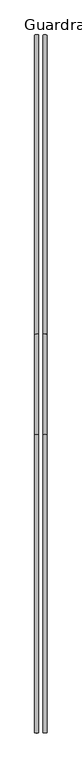
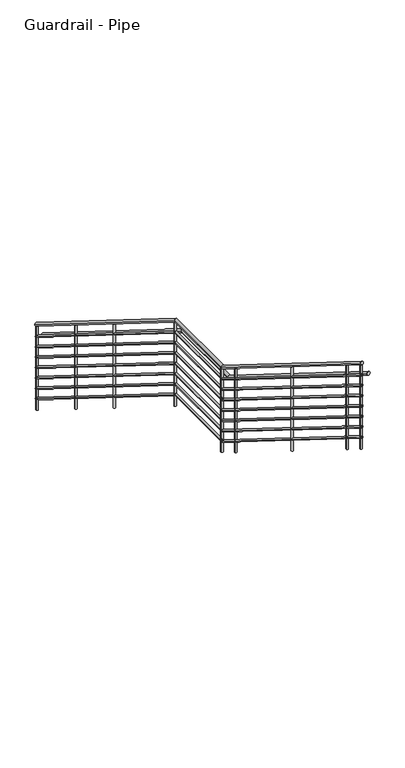
"""IFC4 building model written with IfcOpenShell, lengths in millimetres: railing geometry, Guardrail - Pipe."""

from ifc_helpers import new_model, si_unit, point, frame, frame_2d, origin, place, context, project, spatial, circle_curve, ellipse_curve, trimmed, segment, composite_curve, outline, extrude, source, transform, mapped, element, save
from ifc_brep_helpers import plane_surface, cylinder_surface, advanced_brep


def guardrail_pipe_06b17180(model_context):
    return source(origin(), model_context, "Body", "SolidModel", [
        advanced_brep(
        [(-3343.0939612, 2884.909643, -2439.0768639), (-3304.9939612, 2884.909643, -2439.0768639), (-3343.0939612, 85.4582154, -693.9642857), (-3304.9939612, 85.4582154, -693.9642857), (-3343.0939612, -854.3417846, -693.9642857), (-3304.9939612, -854.3417846, -693.9642857), (-3343.0939612, -3642.890357, 1044.3517075), (-3304.9939612, -3642.890357, 1044.3517075)],
        [
            (0, 1, ellipse_curve(frame((-3324.0439612, 2884.909643, -2439.0768639), z_axis=(0.0, 1.0, 0.0), x_axis=(0.0, 0.0, -1.0)), 22.4482925, 19.05)),
            (1, 0, ellipse_curve(frame((-3324.0439612, 2884.909643, -2439.0768639), z_axis=(0.0, 1.0, 0.0), x_axis=(0.0, 0.0, -1.0)), 22.4482925, 19.05)),
            (0, 2),
            (2, 3, ellipse_curve(frame((-3324.0439612, 85.4582154, -693.9642857), z_axis=(0.0, 0.9614096116045893, -0.2751209892289441), x_axis=(0.0, -0.27512098922894396, -0.9614096116045893)), 19.8146552, 19.05)),
            (3, 1),
            (3, 2, ellipse_curve(frame((-3324.0439612, 85.4582154, -693.9642857), z_axis=(0.0, 0.9614096116045893, -0.2751209892289441), x_axis=(0.0, -0.27512098922894396, -0.9614096116045893)), 19.8146552, 19.05)),
            (2, 4),
            (4, 5, ellipse_curve(frame((-3324.0439612, -854.3417846, -693.9642857), z_axis=(0.0, 0.9614096116045892, -0.27512098922894423), x_axis=(0.0, 0.2751209892289447, 0.9614096116045893)), 19.8146552, 19.05)),
            (5, 3),
            (5, 4, ellipse_curve(frame((-3324.0439612, -854.3417846, -693.9642857), z_axis=(0.0, 0.9614096116045892, -0.27512098922894423), x_axis=(0.0, 0.2751209892289447, 0.9614096116045893)), 19.8146552, 19.05)),
            (6, 7, ellipse_curve(frame((-3324.0439612, -3642.890357, 1044.3517075), z_axis=(0.0, -1.0, 0.0), x_axis=(0.0, 0.0, -1.0)), 22.4482925, 19.05)),
            (7, 6, ellipse_curve(frame((-3324.0439612, -3642.890357, 1044.3517075), z_axis=(0.0, -1.0, 0.0), x_axis=(0.0, 0.0, -1.0)), 22.4482925, 19.05)),
            (4, 6),
            (7, 5),
        ],
        [
            plane_surface(frame((-3324.0439612, 2884.909643, -2416.6285714), z_axis=(0.0, 1.0, 0.0), x_axis=(0.0, 0.0, -1.0))),
            cylinder_surface(frame((-3324.0439612, 2874.832042, -2432.794723), z_axis=(0.0, 0.8486168825713745, -0.5290079267977392), x_axis=(1.0, 0.0, 0.0)), 19.05),
            cylinder_surface(frame((-3324.0439612, 90.909643, -693.9642857), z_axis=(0.0, 1.0, 0.0), x_axis=(1.0, 0.0, 0.0)), 19.05),
            plane_surface(frame((-3324.0439612, -3642.890357, 1066.8), z_axis=(0.0, -1.0, 0.0), x_axis=(0.0, 0.0, -1.0))),
            cylinder_surface(frame((-3324.0439612, -858.967958, -691.0804373), z_axis=(0.0, 0.8486168825713742, -0.5290079267977394), x_axis=(1.0, 0.0, 0.0)), 19.05),
        ],
        [
            (0, [[1, 2]]),
            (1, [[-1, 3, 4, 5]]),
            (1, [[-2, -5, 6, -3]]),
            (2, [[-4, 7, 8, 9]]),
            (2, [[-6, -9, 10, -7]]),
            (3, [[11, 12]]),
            (4, [[-8, 13, -12, 14]]),
            (4, [[-10, -14, -11, -13]]),
        ],
    ),
        advanced_brep(
        [(-3336.7439612, 2884.909643, -2583.9940998), (-3311.3439612, 2884.909643, -2583.9940998), (-3336.7439612, 87.2753579, -840.0142857), (-3311.3439612, 87.2753579, -840.0142857), (-3336.7439612, -852.5246421, -840.0142857), (-3311.3439612, -852.5246421, -840.0142857), (-3336.7439612, -3642.890357, 899.4344717), (-3311.3439612, -3642.890357, 899.4344717)],
        [
            (0, 1, ellipse_curve(frame((-3324.0439612, 2884.909643, -2583.9940998), z_axis=(0.0, 1.0, 0.0), x_axis=(0.0, 0.0, -1.0)), 14.9655283, 12.7)),
            (1, 0, ellipse_curve(frame((-3324.0439612, 2884.909643, -2583.9940998), z_axis=(0.0, 1.0, 0.0), x_axis=(0.0, 0.0, -1.0)), 14.9655283, 12.7)),
            (0, 2),
            (2, 3, ellipse_curve(frame((-3324.0439612, 87.2753579, -840.0142857), z_axis=(0.0, 0.9614096116045893, -0.2751209892289441), x_axis=(0.0, -0.27512098922894396, -0.9614096116045893)), 13.2097702, 12.7)),
            (3, 1),
            (3, 2, ellipse_curve(frame((-3324.0439612, 87.2753579, -840.0142857), z_axis=(0.0, 0.9614096116045893, -0.2751209892289441), x_axis=(0.0, -0.27512098922894396, -0.9614096116045893)), 13.2097702, 12.7)),
            (2, 4),
            (4, 5, ellipse_curve(frame((-3324.0439612, -852.5246421, -840.0142857), z_axis=(0.0, 0.9614096116045892, -0.27512098922894423), x_axis=(0.0, 0.2751209892289447, 0.9614096116045893)), 13.2097702, 12.7)),
            (5, 3),
            (5, 4, ellipse_curve(frame((-3324.0439612, -852.5246421, -840.0142857), z_axis=(0.0, 0.9614096116045892, -0.27512098922894423), x_axis=(0.0, 0.2751209892289447, 0.9614096116045893)), 13.2097702, 12.7)),
            (6, 7, ellipse_curve(frame((-3324.0439612, -3642.890357, 899.4344717), z_axis=(0.0, -1.0, 0.0), x_axis=(0.0, 0.0, -1.0)), 14.9655283, 12.7)),
            (7, 6, ellipse_curve(frame((-3324.0439612, -3642.890357, 899.4344717), z_axis=(0.0, -1.0, 0.0), x_axis=(0.0, 0.0, -1.0)), 14.9655283, 12.7)),
            (4, 6),
            (7, 5),
        ],
        [
            plane_surface(frame((-3324.0439612, 2884.909643, -2569.0285714), z_axis=(0.0, 1.0, 0.0), x_axis=(0.0, 0.0, -1.0))),
            cylinder_surface(frame((-3324.0439612, 2878.1912423, -2579.8060058), z_axis=(0.0, 0.8486168825713745, -0.5290079267977392), x_axis=(1.0, 0.0, 0.0)), 12.7),
            cylinder_surface(frame((-3324.0439612, 90.909643, -840.0142857), z_axis=(0.0, 1.0, 0.0), x_axis=(1.0, 0.0, 0.0)), 12.7),
            plane_surface(frame((-3324.0439612, -3642.890357, 914.4), z_axis=(0.0, -1.0, 0.0), x_axis=(0.0, 0.0, -1.0))),
            cylinder_surface(frame((-3324.0439612, -855.6087577, -838.0917201), z_axis=(0.0, 0.8486168825713742, -0.5290079267977394), x_axis=(1.0, 0.0, 0.0)), 12.7),
        ],
        [
            (0, [[1, 2]]),
            (1, [[-1, 3, 4, 5]]),
            (1, [[-2, -5, 6, -3]]),
            (2, [[-4, 7, 8, 9]]),
            (2, [[-6, -9, 10, -7]]),
            (3, [[11, 12]]),
            (4, [[-8, 13, -12, 14]]),
            (4, [[-10, -14, -11, -13]]),
        ],
    ),
        advanced_brep(
        [(-3266.8939612, 2884.909643, -2591.4768639), (-3228.7939612, 2884.909643, -2591.4768639), (-3266.8939612, 85.4582154, -846.3642857), (-3228.7939612, 85.4582154, -846.3642857), (-3266.8939612, -854.3417846, -846.3642857), (-3228.7939612, -854.3417846, -846.3642857), (-3266.8939612, -3642.890357, 891.9517075), (-3228.7939612, -3642.890357, 891.9517075)],
        [
            (0, 1, ellipse_curve(frame((-3247.8439612, 2884.909643, -2591.4768639), z_axis=(0.0, 1.0, 0.0), x_axis=(0.0, 0.0, -1.0)), 22.4482925, 19.05)),
            (1, 0, ellipse_curve(frame((-3247.8439612, 2884.909643, -2591.4768639), z_axis=(0.0, 1.0, 0.0), x_axis=(0.0, 0.0, -1.0)), 22.4482925, 19.05)),
            (0, 2),
            (2, 3, ellipse_curve(frame((-3247.8439612, 85.4582154, -846.3642857), z_axis=(0.0, 0.9614096116045893, -0.2751209892289441), x_axis=(0.0, -0.27512098922894396, -0.9614096116045893)), 19.8146552, 19.05)),
            (3, 1),
            (3, 2, ellipse_curve(frame((-3247.8439612, 85.4582154, -846.3642857), z_axis=(0.0, 0.9614096116045893, -0.2751209892289441), x_axis=(0.0, -0.27512098922894396, -0.9614096116045893)), 19.8146552, 19.05)),
            (2, 4),
            (4, 5, ellipse_curve(frame((-3247.8439612, -854.3417846, -846.3642857), z_axis=(0.0, 0.9614096116045892, -0.27512098922894423), x_axis=(0.0, 0.2751209892289447, 0.9614096116045893)), 19.8146552, 19.05)),
            (5, 3),
            (5, 4, ellipse_curve(frame((-3247.8439612, -854.3417846, -846.3642857), z_axis=(0.0, 0.9614096116045892, -0.27512098922894423), x_axis=(0.0, 0.2751209892289447, 0.9614096116045893)), 19.8146552, 19.05)),
            (6, 7, ellipse_curve(frame((-3247.8439612, -3642.890357, 891.9517075), z_axis=(0.0, -1.0, 0.0), x_axis=(0.0, 0.0, -1.0)), 22.4482925, 19.05)),
            (7, 6, ellipse_curve(frame((-3247.8439612, -3642.890357, 891.9517075), z_axis=(0.0, -1.0, 0.0), x_axis=(0.0, 0.0, -1.0)), 22.4482925, 19.05)),
            (4, 6),
            (7, 5),
        ],
        [
            plane_surface(frame((-3247.8439612, 2884.909643, -2569.0285714), z_axis=(0.0, 1.0, 0.0), x_axis=(0.0, 0.0, -1.0))),
            cylinder_surface(frame((-3247.8439612, 2874.832042, -2585.194723), z_axis=(0.0, 0.8486168825713745, -0.5290079267977392), x_axis=(1.0, 0.0, 0.0)), 19.05),
            cylinder_surface(frame((-3247.8439612, 90.909643, -846.3642857), z_axis=(0.0, 1.0, 0.0), x_axis=(1.0, 0.0, 0.0)), 19.05),
            plane_surface(frame((-3247.8439612, -3642.890357, 914.4), z_axis=(0.0, -1.0, 0.0), x_axis=(0.0, 0.0, -1.0))),
            cylinder_surface(frame((-3247.8439612, -858.967958, -843.4804373), z_axis=(0.0, 0.8486168825713742, -0.5290079267977394), x_axis=(1.0, 0.0, 0.0)), 19.05),
        ],
        [
            (0, [[1, 2]]),
            (1, [[-1, 3, 4, 5]]),
            (1, [[-2, -5, 6, -3]]),
            (2, [[-4, 7, 8, 9]]),
            (2, [[-6, -9, 10, -7]]),
            (3, [[11, 12]]),
            (4, [[-8, 13, -12, 14]]),
            (4, [[-10, -14, -11, -13]]),
        ],
    ),
        advanced_brep(
        [(-3336.7439612, 2884.909643, -2710.9940998), (-3311.3439612, 2884.909643, -2710.9940998), (-3336.7439612, 87.2753579, -967.0142857), (-3311.3439612, 87.2753579, -967.0142857), (-3336.7439612, -852.5246421, -967.0142857), (-3311.3439612, -852.5246421, -967.0142857), (-3336.7439612, -3642.890357, 772.4344717), (-3311.3439612, -3642.890357, 772.4344717)],
        [
            (0, 1, ellipse_curve(frame((-3324.0439612, 2884.909643, -2710.9940998), z_axis=(0.0, 1.0, 0.0), x_axis=(0.0, 0.0, -1.0)), 14.9655283, 12.7)),
            (1, 0, ellipse_curve(frame((-3324.0439612, 2884.909643, -2710.9940998), z_axis=(0.0, 1.0, 0.0), x_axis=(0.0, 0.0, -1.0)), 14.9655283, 12.7)),
            (0, 2),
            (2, 3, ellipse_curve(frame((-3324.0439612, 87.2753579, -967.0142857), z_axis=(0.0, 0.9614096116045893, -0.2751209892289441), x_axis=(0.0, -0.27512098922894396, -0.9614096116045893)), 13.2097702, 12.7)),
            (3, 1),
            (3, 2, ellipse_curve(frame((-3324.0439612, 87.2753579, -967.0142857), z_axis=(0.0, 0.9614096116045893, -0.2751209892289441), x_axis=(0.0, -0.27512098922894396, -0.9614096116045893)), 13.2097702, 12.7)),
            (2, 4),
            (4, 5, ellipse_curve(frame((-3324.0439612, -852.5246421, -967.0142857), z_axis=(0.0, 0.9614096116045892, -0.27512098922894423), x_axis=(0.0, 0.2751209892289447, 0.9614096116045893)), 13.2097702, 12.7)),
            (5, 3),
            (5, 4, ellipse_curve(frame((-3324.0439612, -852.5246421, -967.0142857), z_axis=(0.0, 0.9614096116045892, -0.27512098922894423), x_axis=(0.0, 0.2751209892289447, 0.9614096116045893)), 13.2097702, 12.7)),
            (6, 7, ellipse_curve(frame((-3324.0439612, -3642.890357, 772.4344717), z_axis=(0.0, -1.0, 0.0), x_axis=(0.0, 0.0, -1.0)), 14.9655283, 12.7)),
            (7, 6, ellipse_curve(frame((-3324.0439612, -3642.890357, 772.4344717), z_axis=(0.0, -1.0, 0.0), x_axis=(0.0, 0.0, -1.0)), 14.9655283, 12.7)),
            (4, 6),
            (7, 5),
        ],
        [
            plane_surface(frame((-3324.0439612, 2884.909643, -2696.0285714), z_axis=(0.0, 1.0, 0.0), x_axis=(0.0, 0.0, -1.0))),
            cylinder_surface(frame((-3324.0439612, 2878.1912423, -2706.8060058), z_axis=(0.0, 0.8486168825713745, -0.5290079267977392), x_axis=(1.0, 0.0, 0.0)), 12.7),
            cylinder_surface(frame((-3324.0439612, 90.909643, -967.0142857), z_axis=(0.0, 1.0, 0.0), x_axis=(1.0, 0.0, 0.0)), 12.7),
            plane_surface(frame((-3324.0439612, -3642.890357, 787.4), z_axis=(0.0, -1.0, 0.0), x_axis=(0.0, 0.0, -1.0))),
            cylinder_surface(frame((-3324.0439612, -855.6087577, -965.0917201), z_axis=(0.0, 0.8486168825713742, -0.5290079267977394), x_axis=(1.0, 0.0, 0.0)), 12.7),
        ],
        [
            (0, [[1, 2]]),
            (1, [[-1, 3, 4, 5]]),
            (1, [[-2, -5, 6, -3]]),
            (2, [[-4, 7, 8, 9]]),
            (2, [[-6, -9, 10, -7]]),
            (3, [[11, 12]]),
            (4, [[-8, 13, -12, 14]]),
            (4, [[-10, -14, -11, -13]]),
        ],
    ),
        advanced_brep(
        [(-3336.7439612, 2884.909643, -2837.9940998), (-3311.3439612, 2884.909643, -2837.9940998), (-3336.7439612, 87.2753579, -1094.0142857), (-3311.3439612, 87.2753579, -1094.0142857), (-3336.7439612, -852.5246421, -1094.0142857), (-3311.3439612, -852.5246421, -1094.0142857), (-3336.7439612, -3642.890357, 645.4344717), (-3311.3439612, -3642.890357, 645.4344717)],
        [
            (0, 1, ellipse_curve(frame((-3324.0439612, 2884.909643, -2837.9940998), z_axis=(0.0, 1.0, 0.0), x_axis=(0.0, 0.0, -1.0)), 14.9655283, 12.7)),
            (1, 0, ellipse_curve(frame((-3324.0439612, 2884.909643, -2837.9940998), z_axis=(0.0, 1.0, 0.0), x_axis=(0.0, 0.0, -1.0)), 14.9655283, 12.7)),
            (0, 2),
            (2, 3, ellipse_curve(frame((-3324.0439612, 87.2753579, -1094.0142857), z_axis=(0.0, 0.9614096116045893, -0.2751209892289441), x_axis=(0.0, -0.27512098922894396, -0.9614096116045893)), 13.2097702, 12.7)),
            (3, 1),
            (3, 2, ellipse_curve(frame((-3324.0439612, 87.2753579, -1094.0142857), z_axis=(0.0, 0.9614096116045893, -0.2751209892289441), x_axis=(0.0, -0.27512098922894396, -0.9614096116045893)), 13.2097702, 12.7)),
            (2, 4),
            (4, 5, ellipse_curve(frame((-3324.0439612, -852.5246421, -1094.0142857), z_axis=(0.0, 0.9614096116045892, -0.27512098922894423), x_axis=(0.0, 0.2751209892289447, 0.9614096116045893)), 13.2097702, 12.7)),
            (5, 3),
            (5, 4, ellipse_curve(frame((-3324.0439612, -852.5246421, -1094.0142857), z_axis=(0.0, 0.9614096116045892, -0.27512098922894423), x_axis=(0.0, 0.2751209892289447, 0.9614096116045893)), 13.2097702, 12.7)),
            (6, 7, ellipse_curve(frame((-3324.0439612, -3642.890357, 645.4344717), z_axis=(0.0, -1.0, 0.0), x_axis=(0.0, 0.0, -1.0)), 14.9655283, 12.7)),
            (7, 6, ellipse_curve(frame((-3324.0439612, -3642.890357, 645.4344717), z_axis=(0.0, -1.0, 0.0), x_axis=(0.0, 0.0, -1.0)), 14.9655283, 12.7)),
            (4, 6),
            (7, 5),
        ],
        [
            plane_surface(frame((-3324.0439612, 2884.909643, -2823.0285714), z_axis=(0.0, 1.0, 0.0), x_axis=(0.0, 0.0, -1.0))),
            cylinder_surface(frame((-3324.0439612, 2878.1912423, -2833.8060058), z_axis=(0.0, 0.8486168825713745, -0.5290079267977392), x_axis=(1.0, 0.0, 0.0)), 12.7),
            cylinder_surface(frame((-3324.0439612, 90.909643, -1094.0142857), z_axis=(0.0, 1.0, 0.0), x_axis=(1.0, 0.0, 0.0)), 12.7),
            plane_surface(frame((-3324.0439612, -3642.890357, 660.4), z_axis=(0.0, -1.0, 0.0), x_axis=(0.0, 0.0, -1.0))),
            cylinder_surface(frame((-3324.0439612, -855.6087577, -1092.0917201), z_axis=(0.0, 0.8486168825713742, -0.5290079267977394), x_axis=(1.0, 0.0, 0.0)), 12.7),
        ],
        [
            (0, [[1, 2]]),
            (1, [[-1, 3, 4, 5]]),
            (1, [[-2, -5, 6, -3]]),
            (2, [[-4, 7, 8, 9]]),
            (2, [[-6, -9, 10, -7]]),
            (3, [[11, 12]]),
            (4, [[-8, 13, -12, 14]]),
            (4, [[-10, -14, -11, -13]]),
        ],
    ),
        advanced_brep(
        [(-3336.7439612, 2884.909643, -2964.9940998), (-3311.3439612, 2884.909643, -2964.9940998), (-3336.7439612, 87.2753579, -1221.0142857), (-3311.3439612, 87.2753579, -1221.0142857), (-3336.7439612, -852.5246421, -1221.0142857), (-3311.3439612, -852.5246421, -1221.0142857), (-3336.7439612, -3642.890357, 518.4344717), (-3311.3439612, -3642.890357, 518.4344717)],
        [
            (0, 1, ellipse_curve(frame((-3324.0439612, 2884.909643, -2964.9940998), z_axis=(0.0, 1.0, 0.0), x_axis=(0.0, 0.0, -1.0)), 14.9655283, 12.7)),
            (1, 0, ellipse_curve(frame((-3324.0439612, 2884.909643, -2964.9940998), z_axis=(0.0, 1.0, 0.0), x_axis=(0.0, 0.0, -1.0)), 14.9655283, 12.7)),
            (0, 2),
            (2, 3, ellipse_curve(frame((-3324.0439612, 87.2753579, -1221.0142857), z_axis=(0.0, 0.9614096116045893, -0.2751209892289441), x_axis=(0.0, -0.27512098922894396, -0.9614096116045893)), 13.2097702, 12.7)),
            (3, 1),
            (3, 2, ellipse_curve(frame((-3324.0439612, 87.2753579, -1221.0142857), z_axis=(0.0, 0.9614096116045893, -0.2751209892289441), x_axis=(0.0, -0.27512098922894396, -0.9614096116045893)), 13.2097702, 12.7)),
            (2, 4),
            (4, 5, ellipse_curve(frame((-3324.0439612, -852.5246421, -1221.0142857), z_axis=(0.0, 0.9614096116045892, -0.27512098922894423), x_axis=(0.0, 0.2751209892289447, 0.9614096116045893)), 13.2097702, 12.7)),
            (5, 3),
            (5, 4, ellipse_curve(frame((-3324.0439612, -852.5246421, -1221.0142857), z_axis=(0.0, 0.9614096116045892, -0.27512098922894423), x_axis=(0.0, 0.2751209892289447, 0.9614096116045893)), 13.2097702, 12.7)),
            (6, 7, ellipse_curve(frame((-3324.0439612, -3642.890357, 518.4344717), z_axis=(0.0, -1.0, 0.0), x_axis=(0.0, 0.0, -1.0)), 14.9655283, 12.7)),
            (7, 6, ellipse_curve(frame((-3324.0439612, -3642.890357, 518.4344717), z_axis=(0.0, -1.0, 0.0), x_axis=(0.0, 0.0, -1.0)), 14.9655283, 12.7)),
            (4, 6),
            (7, 5),
        ],
        [
            plane_surface(frame((-3324.0439612, 2884.909643, -2950.0285714), z_axis=(0.0, 1.0, 0.0), x_axis=(0.0, 0.0, -1.0))),
            cylinder_surface(frame((-3324.0439612, 2878.1912423, -2960.8060058), z_axis=(0.0, 0.8486168825713745, -0.5290079267977392), x_axis=(1.0, 0.0, 0.0)), 12.7),
            cylinder_surface(frame((-3324.0439612, 90.909643, -1221.0142857), z_axis=(0.0, 1.0, 0.0), x_axis=(1.0, 0.0, 0.0)), 12.7),
            plane_surface(frame((-3324.0439612, -3642.890357, 533.4), z_axis=(0.0, -1.0, 0.0), x_axis=(0.0, 0.0, -1.0))),
            cylinder_surface(frame((-3324.0439612, -855.6087577, -1219.0917201), z_axis=(0.0, 0.8486168825713742, -0.5290079267977394), x_axis=(1.0, 0.0, 0.0)), 12.7),
        ],
        [
            (0, [[1, 2]]),
            (1, [[-1, 3, 4, 5]]),
            (1, [[-2, -5, 6, -3]]),
            (2, [[-4, 7, 8, 9]]),
            (2, [[-6, -9, 10, -7]]),
            (3, [[11, 12]]),
            (4, [[-8, 13, -12, 14]]),
            (4, [[-10, -14, -11, -13]]),
        ],
    ),
        advanced_brep(
        [(-3336.7439612, 2884.909643, -3091.9940998), (-3311.3439612, 2884.909643, -3091.9940998), (-3336.7439612, 87.2753579, -1348.0142857), (-3311.3439612, 87.2753579, -1348.0142857), (-3336.7439612, -852.5246421, -1348.0142857), (-3311.3439612, -852.5246421, -1348.0142857), (-3336.7439612, -3642.890357, 391.4344717), (-3311.3439612, -3642.890357, 391.4344717)],
        [
            (0, 1, ellipse_curve(frame((-3324.0439612, 2884.909643, -3091.9940998), z_axis=(0.0, 1.0, 0.0), x_axis=(0.0, 0.0, -1.0)), 14.9655283, 12.7)),
            (1, 0, ellipse_curve(frame((-3324.0439612, 2884.909643, -3091.9940998), z_axis=(0.0, 1.0, 0.0), x_axis=(0.0, 0.0, -1.0)), 14.9655283, 12.7)),
            (0, 2),
            (2, 3, ellipse_curve(frame((-3324.0439612, 87.2753579, -1348.0142857), z_axis=(0.0, 0.9614096116045893, -0.2751209892289441), x_axis=(0.0, -0.27512098922894396, -0.9614096116045893)), 13.2097702, 12.7)),
            (3, 1),
            (3, 2, ellipse_curve(frame((-3324.0439612, 87.2753579, -1348.0142857), z_axis=(0.0, 0.9614096116045893, -0.2751209892289441), x_axis=(0.0, -0.27512098922894396, -0.9614096116045893)), 13.2097702, 12.7)),
            (2, 4),
            (4, 5, ellipse_curve(frame((-3324.0439612, -852.5246421, -1348.0142857), z_axis=(0.0, 0.9614096116045892, -0.27512098922894423), x_axis=(0.0, 0.2751209892289447, 0.9614096116045893)), 13.2097702, 12.7)),
            (5, 3),
            (5, 4, ellipse_curve(frame((-3324.0439612, -852.5246421, -1348.0142857), z_axis=(0.0, 0.9614096116045892, -0.27512098922894423), x_axis=(0.0, 0.2751209892289447, 0.9614096116045893)), 13.2097702, 12.7)),
            (6, 7, ellipse_curve(frame((-3324.0439612, -3642.890357, 391.4344717), z_axis=(0.0, -1.0, 0.0), x_axis=(0.0, 0.0, -1.0)), 14.9655283, 12.7)),
            (7, 6, ellipse_curve(frame((-3324.0439612, -3642.890357, 391.4344717), z_axis=(0.0, -1.0, 0.0), x_axis=(0.0, 0.0, -1.0)), 14.9655283, 12.7)),
            (4, 6),
            (7, 5),
        ],
        [
            plane_surface(frame((-3324.0439612, 2884.909643, -3077.0285714), z_axis=(0.0, 1.0, 0.0), x_axis=(0.0, 0.0, -1.0))),
            cylinder_surface(frame((-3324.0439612, 2878.1912423, -3087.8060058), z_axis=(0.0, 0.8486168825713745, -0.5290079267977392), x_axis=(1.0, 0.0, 0.0)), 12.7),
            cylinder_surface(frame((-3324.0439612, 90.909643, -1348.0142857), z_axis=(0.0, 1.0, 0.0), x_axis=(1.0, 0.0, 0.0)), 12.7),
            plane_surface(frame((-3324.0439612, -3642.890357, 406.4), z_axis=(0.0, -1.0, 0.0), x_axis=(0.0, 0.0, -1.0))),
            cylinder_surface(frame((-3324.0439612, -855.6087577, -1346.0917201), z_axis=(0.0, 0.8486168825713742, -0.5290079267977394), x_axis=(1.0, 0.0, 0.0)), 12.7),
        ],
        [
            (0, [[1, 2]]),
            (1, [[-1, 3, 4, 5]]),
            (1, [[-2, -5, 6, -3]]),
            (2, [[-4, 7, 8, 9]]),
            (2, [[-6, -9, 10, -7]]),
            (3, [[11, 12]]),
            (4, [[-8, 13, -12, 14]]),
            (4, [[-10, -14, -11, -13]]),
        ],
    ),
        advanced_brep(
        [(-3336.7439612, 2884.909643, -3218.9940998), (-3311.3439612, 2884.909643, -3218.9940998), (-3336.7439612, 87.2753579, -1475.0142857), (-3311.3439612, 87.2753579, -1475.0142857), (-3336.7439612, -852.5246421, -1475.0142857), (-3311.3439612, -852.5246421, -1475.0142857), (-3336.7439612, -3642.890357, 264.4344717), (-3311.3439612, -3642.890357, 264.4344717)],
        [
            (0, 1, ellipse_curve(frame((-3324.0439612, 2884.909643, -3218.9940998), z_axis=(0.0, 1.0, 0.0), x_axis=(0.0, 0.0, -1.0)), 14.9655283, 12.7)),
            (1, 0, ellipse_curve(frame((-3324.0439612, 2884.909643, -3218.9940998), z_axis=(0.0, 1.0, 0.0), x_axis=(0.0, 0.0, -1.0)), 14.9655283, 12.7)),
            (0, 2),
            (2, 3, ellipse_curve(frame((-3324.0439612, 87.2753579, -1475.0142857), z_axis=(0.0, 0.9614096116045893, -0.2751209892289441), x_axis=(0.0, -0.27512098922894396, -0.9614096116045893)), 13.2097702, 12.7)),
            (3, 1),
            (3, 2, ellipse_curve(frame((-3324.0439612, 87.2753579, -1475.0142857), z_axis=(0.0, 0.9614096116045893, -0.2751209892289441), x_axis=(0.0, -0.27512098922894396, -0.9614096116045893)), 13.2097702, 12.7)),
            (2, 4),
            (4, 5, ellipse_curve(frame((-3324.0439612, -852.5246421, -1475.0142857), z_axis=(0.0, 0.9614096116045892, -0.27512098922894423), x_axis=(0.0, 0.2751209892289447, 0.9614096116045893)), 13.2097702, 12.7)),
            (5, 3),
            (5, 4, ellipse_curve(frame((-3324.0439612, -852.5246421, -1475.0142857), z_axis=(0.0, 0.9614096116045892, -0.27512098922894423), x_axis=(0.0, 0.2751209892289447, 0.9614096116045893)), 13.2097702, 12.7)),
            (6, 7, ellipse_curve(frame((-3324.0439612, -3642.890357, 264.4344717), z_axis=(0.0, -1.0, 0.0), x_axis=(0.0, 0.0, -1.0)), 14.9655283, 12.7)),
            (7, 6, ellipse_curve(frame((-3324.0439612, -3642.890357, 264.4344717), z_axis=(0.0, -1.0, 0.0), x_axis=(0.0, 0.0, -1.0)), 14.9655283, 12.7)),
            (4, 6),
            (7, 5),
        ],
        [
            plane_surface(frame((-3324.0439612, 2884.909643, -3204.0285714), z_axis=(0.0, 1.0, 0.0), x_axis=(0.0, 0.0, -1.0))),
            cylinder_surface(frame((-3324.0439612, 2878.1912423, -3214.8060058), z_axis=(0.0, 0.8486168825713745, -0.5290079267977392), x_axis=(1.0, 0.0, 0.0)), 12.7),
            cylinder_surface(frame((-3324.0439612, 90.909643, -1475.0142857), z_axis=(0.0, 1.0, 0.0), x_axis=(1.0, 0.0, 0.0)), 12.7),
            plane_surface(frame((-3324.0439612, -3642.890357, 279.4), z_axis=(0.0, -1.0, 0.0), x_axis=(0.0, 0.0, -1.0))),
            cylinder_surface(frame((-3324.0439612, -855.6087577, -1473.0917201), z_axis=(0.0, 0.8486168825713742, -0.5290079267977394), x_axis=(1.0, 0.0, 0.0)), 12.7),
        ],
        [
            (0, [[1, 2]]),
            (1, [[-1, 3, 4, 5]]),
            (1, [[-2, -5, 6, -3]]),
            (2, [[-4, 7, 8, 9]]),
            (2, [[-6, -9, 10, -7]]),
            (3, [[11, 12]]),
            (4, [[-8, 13, -12, 14]]),
            (4, [[-10, -14, -11, -13]]),
        ],
    ),
        advanced_brep(
        [(-3336.7439612, 2884.909643, -3345.9940998), (-3311.3439612, 2884.909643, -3345.9940998), (-3336.7439612, 87.2753579, -1602.0142857), (-3311.3439612, 87.2753579, -1602.0142857), (-3336.7439612, -852.5246421, -1602.0142857), (-3311.3439612, -852.5246421, -1602.0142857), (-3336.7439612, -3642.890357, 137.4344717), (-3311.3439612, -3642.890357, 137.4344717)],
        [
            (0, 1, ellipse_curve(frame((-3324.0439612, 2884.909643, -3345.9940998), z_axis=(0.0, 1.0, 0.0), x_axis=(0.0, 0.0, -1.0)), 14.9655283, 12.7)),
            (1, 0, ellipse_curve(frame((-3324.0439612, 2884.909643, -3345.9940998), z_axis=(0.0, 1.0, 0.0), x_axis=(0.0, 0.0, -1.0)), 14.9655283, 12.7)),
            (0, 2),
            (2, 3, ellipse_curve(frame((-3324.0439612, 87.2753579, -1602.0142857), z_axis=(0.0, 0.9614096116045893, -0.2751209892289441), x_axis=(0.0, -0.27512098922894396, -0.9614096116045893)), 13.2097702, 12.7)),
            (3, 1),
            (3, 2, ellipse_curve(frame((-3324.0439612, 87.2753579, -1602.0142857), z_axis=(0.0, 0.9614096116045893, -0.2751209892289441), x_axis=(0.0, -0.27512098922894396, -0.9614096116045893)), 13.2097702, 12.7)),
            (2, 4),
            (4, 5, ellipse_curve(frame((-3324.0439612, -852.5246421, -1602.0142857), z_axis=(0.0, 0.9614096116045892, -0.27512098922894423), x_axis=(0.0, 0.2751209892289447, 0.9614096116045893)), 13.2097702, 12.7)),
            (5, 3),
            (5, 4, ellipse_curve(frame((-3324.0439612, -852.5246421, -1602.0142857), z_axis=(0.0, 0.9614096116045892, -0.27512098922894423), x_axis=(0.0, 0.2751209892289447, 0.9614096116045893)), 13.2097702, 12.7)),
            (6, 7, ellipse_curve(frame((-3324.0439612, -3642.890357, 137.4344717), z_axis=(0.0, -1.0, 0.0), x_axis=(0.0, 0.0, -1.0)), 14.9655283, 12.7)),
            (7, 6, ellipse_curve(frame((-3324.0439612, -3642.890357, 137.4344717), z_axis=(0.0, -1.0, 0.0), x_axis=(0.0, 0.0, -1.0)), 14.9655283, 12.7)),
            (4, 6),
            (7, 5),
        ],
        [
            plane_surface(frame((-3324.0439612, 2884.909643, -3331.0285714), z_axis=(0.0, 1.0, 0.0), x_axis=(0.0, 0.0, -1.0))),
            cylinder_surface(frame((-3324.0439612, 2878.1912423, -3341.8060058), z_axis=(0.0, 0.8486168825713745, -0.5290079267977392), x_axis=(1.0, 0.0, 0.0)), 12.7),
            cylinder_surface(frame((-3324.0439612, 90.909643, -1602.0142857), z_axis=(0.0, 1.0, 0.0), x_axis=(1.0, 0.0, 0.0)), 12.7),
            plane_surface(frame((-3324.0439612, -3642.890357, 152.4), z_axis=(0.0, -1.0, 0.0), x_axis=(0.0, 0.0, -1.0))),
            cylinder_surface(frame((-3324.0439612, -855.6087577, -1600.0917201), z_axis=(0.0, 0.8486168825713742, -0.5290079267977394), x_axis=(1.0, 0.0, 0.0)), 12.7),
        ],
        [
            (0, [[1, 2]]),
            (1, [[-1, 3, 4, 5]]),
            (1, [[-2, -5, 6, -3]]),
            (2, [[-4, 7, 8, 9]]),
            (2, [[-6, -9, 10, -7]]),
            (3, [[11, 12]]),
            (4, [[-8, 13, -12, 14]]),
            (4, [[-10, -14, -11, -13]]),
        ],
    ),
        advanced_brep(
        [(-3336.7439612, -3630.5087726, -7.7183903), (-3311.3439612, -3630.5087726, -7.7183903), (-3311.3439612, -3630.5087726, 1014.1850247), (-3336.7439612, -3630.5087726, 1014.1850247)],
        [
            (0, 1, circle_curve(frame((-3324.0439612, -3630.5087726, -7.7183903), z_axis=(0.0, 0.0, -1.0), x_axis=(1.0, 0.0, 0.0)), 12.7)),
            (1, 0, circle_curve(frame((-3324.0439612, -3630.5087726, -7.7183903), z_axis=(0.0, 0.0, -1.0), x_axis=(1.0, 0.0, 0.0)), 12.7)),
            (1, 2),
            (2, 3, ellipse_curve(frame((-3324.0439612, -3630.5087726, 1014.1850247), z_axis=(0.0, -0.5290079267977408, -0.8486168825713734), x_axis=(0.0, -0.8486168825713732, 0.5290079267977408)), 14.9655283, 12.7)),
            (3, 0),
            (3, 2, ellipse_curve(frame((-3324.0439612, -3630.5087726, 1014.1850247), z_axis=(0.0, -0.5290079267977408, -0.8486168825713734), x_axis=(0.0, -0.8486168825713732, 0.5290079267977408)), 14.9655283, 12.7)),
        ],
        [
            plane_surface(frame((-3311.3439612, -3630.5087726, -7.7183903), z_axis=(0.0, 0.0, -1.0), x_axis=(0.0, -1.0, 0.0))),
            cylinder_surface(frame((-3324.0439612, -3630.5087726, -7.7183903), z_axis=(0.0, 0.0, 1.0), x_axis=(1.0, 0.0, 0.0)), 12.7),
            plane_surface(frame((-3276.8181313, -3665.4337726, 1035.9564532), z_axis=(0.0, 0.5290079267977408, 0.8486168825713734), x_axis=(-1.0, 0.0, 0.0))),
        ],
        [
            (0, [[1, 2]]),
            (1, [[-2, 3, 4, 5]]),
            (1, [[-1, -5, 6, -3]]),
            (2, [[-4, -6]]),
        ],
    ),
        advanced_brep(
        [(-3336.7439612, -3351.1087726, -181.8898189), (-3311.3439612, -3351.1087726, -181.8898189), (-3311.3439612, -3351.1087726, 840.0135961), (-3336.7439612, -3351.1087726, 840.0135961)],
        [
            (0, 1, circle_curve(frame((-3324.0439612, -3351.1087726, -181.8898189), z_axis=(0.0, 0.0, -1.0), x_axis=(1.0, 0.0, 0.0)), 12.7)),
            (1, 0, circle_curve(frame((-3324.0439612, -3351.1087726, -181.8898189), z_axis=(0.0, 0.0, -1.0), x_axis=(1.0, 0.0, 0.0)), 12.7)),
            (1, 2),
            (2, 3, ellipse_curve(frame((-3324.0439612, -3351.1087726, 840.0135961), z_axis=(0.0, -0.5290079267977408, -0.8486168825713734), x_axis=(0.0, -0.8486168825713732, 0.5290079267977408)), 14.9655283, 12.7)),
            (3, 0),
            (3, 2, ellipse_curve(frame((-3324.0439612, -3351.1087726, 840.0135961), z_axis=(0.0, -0.5290079267977408, -0.8486168825713734), x_axis=(0.0, -0.8486168825713732, 0.5290079267977408)), 14.9655283, 12.7)),
        ],
        [
            plane_surface(frame((-3311.3439612, -3351.1087726, -181.8898189), z_axis=(0.0, 0.0, -1.0), x_axis=(0.0, -1.0, 0.0))),
            cylinder_surface(frame((-3324.0439612, -3351.1087726, -181.8898189), z_axis=(0.0, 0.0, 1.0), x_axis=(1.0, 0.0, 0.0)), 12.7),
            plane_surface(frame((-3276.8181313, -3386.0337726, 861.7850247), z_axis=(0.0, 0.5290079267977408, 0.8486168825713734), x_axis=(-1.0, 0.0, 0.0))),
        ],
        [
            (0, [[1, 2]]),
            (1, [[-2, 3, 4, 5]]),
            (1, [[-1, -5, 6, -3]]),
            (2, [[-4, -6]]),
        ],
    ),
        advanced_brep(
        [(-3336.7439612, -2245.890357, -870.8571429), (-3311.3439612, -2245.890357, -870.8571429), (-3311.3439612, -2245.890357, 151.0462721), (-3336.7439612, -2245.890357, 151.0462721)],
        [
            (0, 1, circle_curve(frame((-3324.0439612, -2245.890357, -870.8571429), z_axis=(0.0, 0.0, -1.0), x_axis=(1.0, 0.0, 0.0)), 12.7)),
            (1, 0, circle_curve(frame((-3324.0439612, -2245.890357, -870.8571429), z_axis=(0.0, 0.0, -1.0), x_axis=(1.0, 0.0, 0.0)), 12.7)),
            (1, 2),
            (2, 3, ellipse_curve(frame((-3324.0439612, -2245.890357, 151.0462721), z_axis=(0.0, -0.5290079267977408, -0.8486168825713734), x_axis=(0.0, -0.8486168825713732, 0.5290079267977408)), 14.9655283, 12.7)),
            (3, 0),
            (3, 2, ellipse_curve(frame((-3324.0439612, -2245.890357, 151.0462721), z_axis=(0.0, -0.5290079267977408, -0.8486168825713734), x_axis=(0.0, -0.8486168825713732, 0.5290079267977408)), 14.9655283, 12.7)),
        ],
        [
            plane_surface(frame((-3311.3439612, -2245.890357, -870.8571429), z_axis=(0.0, 0.0, -1.0), x_axis=(0.0, -1.0, 0.0))),
            cylinder_surface(frame((-3324.0439612, -2245.890357, -870.8571429), z_axis=(0.0, 0.0, 1.0), x_axis=(1.0, 0.0, 0.0)), 12.7),
            plane_surface(frame((-3276.8181313, -2280.815357, 172.8177007), z_axis=(0.0, 0.5290079267977408, 0.8486168825713734), x_axis=(-1.0, 0.0, 0.0))),
        ],
        [
            (0, [[1, 2]]),
            (1, [[-2, 3, 4, 5]]),
            (1, [[-1, -5, 6, -3]]),
            (2, [[-4, -6]]),
        ],
    ),
        advanced_brep(
        [(-3336.7439612, -1115.9087726, -1575.2612475), (-3311.3439612, -1115.9087726, -1575.2612475), (-3311.3439612, -1115.9087726, -553.3578325), (-3336.7439612, -1115.9087726, -553.3578325)],
        [
            (0, 1, circle_curve(frame((-3324.0439612, -1115.9087726, -1575.2612475), z_axis=(0.0, 0.0, -1.0), x_axis=(1.0, 0.0, 0.0)), 12.7)),
            (1, 0, circle_curve(frame((-3324.0439612, -1115.9087726, -1575.2612475), z_axis=(0.0, 0.0, -1.0), x_axis=(1.0, 0.0, 0.0)), 12.7)),
            (1, 2),
            (2, 3, ellipse_curve(frame((-3324.0439612, -1115.9087726, -553.3578325), z_axis=(0.0, -0.5290079267977408, -0.8486168825713734), x_axis=(0.0, -0.8486168825713732, 0.5290079267977408)), 14.9655283, 12.7)),
            (3, 0),
            (3, 2, ellipse_curve(frame((-3324.0439612, -1115.9087726, -553.3578325), z_axis=(0.0, -0.5290079267977408, -0.8486168825713734), x_axis=(0.0, -0.8486168825713732, 0.5290079267977408)), 14.9655283, 12.7)),
        ],
        [
            plane_surface(frame((-3311.3439612, -1115.9087726, -1575.2612475), z_axis=(0.0, 0.0, -1.0), x_axis=(0.0, -1.0, 0.0))),
            cylinder_surface(frame((-3324.0439612, -1115.9087726, -1575.2612475), z_axis=(0.0, 0.0, 1.0), x_axis=(1.0, 0.0, 0.0)), 12.7),
            plane_surface(frame((-3276.8181313, -1150.8337726, -531.5864039), z_axis=(0.0, 0.5290079267977408, 0.8486168825713734), x_axis=(-1.0, 0.0, 0.0))),
        ],
        [
            (0, [[1, 2]]),
            (1, [[-2, 3, 4, 5]]),
            (1, [[-1, -5, 6, -3]]),
            (2, [[-4, -6]]),
        ],
    ),
        extrude(outline(composite_curve([segment(trimmed(circle_curve(frame_2d((-3324.0439612, -836.5087726)), 12.7), [point((-3336.7439612, -836.5087726))], [point((-3311.3439612, -836.5087726))], False, "CARTESIAN"), True, "CONTINUOUS"), segment(trimmed(circle_curve(frame_2d((-3324.0439612, -836.5087726)), 12.7), [point((-3311.3439612, -836.5087726))], [point((-3336.7439612, -836.5087726))], False, "CARTESIAN"), True, "CONTINUOUS")], self_intersect=False)), frame((0.0, 0.0, -1741.7142857), z_axis=(0.0, 0.0, 1.0), x_axis=(1.0, 0.0, 0.0)), (0.0, 0.0, 1.0), 1028.7),
        advanced_brep(
        [(-3336.7439612, 103.2912274, -1749.432676), (-3311.3439612, 103.2912274, -1749.432676), (-3311.3439612, 103.2912274, -727.529261), (-3336.7439612, 103.2912274, -727.529261)],
        [
            (0, 1, circle_curve(frame((-3324.0439612, 103.2912274, -1749.432676), z_axis=(0.0, 0.0, -1.0), x_axis=(1.0, 0.0, 0.0)), 12.7)),
            (1, 0, circle_curve(frame((-3324.0439612, 103.2912274, -1749.432676), z_axis=(0.0, 0.0, -1.0), x_axis=(1.0, 0.0, 0.0)), 12.7)),
            (1, 2),
            (2, 3, ellipse_curve(frame((-3324.0439612, 103.2912274, -727.529261), z_axis=(0.0, -0.5290079267977408, -0.8486168825713734), x_axis=(0.0, -0.8486168825713732, 0.5290079267977408)), 14.9655283, 12.7)),
            (3, 0),
            (3, 2, ellipse_curve(frame((-3324.0439612, 103.2912274, -727.529261), z_axis=(0.0, -0.5290079267977408, -0.8486168825713734), x_axis=(0.0, -0.8486168825713732, 0.5290079267977408)), 14.9655283, 12.7)),
        ],
        [
            plane_surface(frame((-3311.3439612, 103.2912274, -1749.432676), z_axis=(0.0, 0.0, -1.0), x_axis=(0.0, -1.0, 0.0))),
            cylinder_surface(frame((-3324.0439612, 103.2912274, -1749.432676), z_axis=(0.0, 0.0, 1.0), x_axis=(1.0, 0.0, 0.0)), 12.7),
            plane_surface(frame((-3276.8181313, 68.3662274, -705.7578325), z_axis=(0.0, 0.5290079267977408, 0.8486168825713734), x_axis=(-1.0, 0.0, 0.0))),
        ],
        [
            (0, [[1, 2]]),
            (1, [[-2, 3, 4, 5]]),
            (1, [[-1, -5, 6, -3]]),
            (2, [[-4, -6]]),
        ],
    ),
        advanced_brep(
        [(-3336.7439612, 1322.4912274, -2509.4534553), (-3311.3439612, 1322.4912274, -2509.4534553), (-3311.3439612, 1322.4912274, -1487.5500403), (-3336.7439612, 1322.4912274, -1487.5500403)],
        [
            (0, 1, circle_curve(frame((-3324.0439612, 1322.4912274, -2509.4534553), z_axis=(0.0, 0.0, -1.0), x_axis=(1.0, 0.0, 0.0)), 12.7)),
            (1, 0, circle_curve(frame((-3324.0439612, 1322.4912274, -2509.4534553), z_axis=(0.0, 0.0, -1.0), x_axis=(1.0, 0.0, 0.0)), 12.7)),
            (1, 2),
            (2, 3, ellipse_curve(frame((-3324.0439612, 1322.4912274, -1487.5500403), z_axis=(0.0, -0.5290079267977408, -0.8486168825713734), x_axis=(0.0, -0.8486168825713732, 0.5290079267977408)), 14.9655283, 12.7)),
            (3, 0),
            (3, 2, ellipse_curve(frame((-3324.0439612, 1322.4912274, -1487.5500403), z_axis=(0.0, -0.5290079267977408, -0.8486168825713734), x_axis=(0.0, -0.8486168825713732, 0.5290079267977408)), 14.9655283, 12.7)),
        ],
        [
            plane_surface(frame((-3311.3439612, 1322.4912274, -2509.4534553), z_axis=(0.0, 0.0, -1.0), x_axis=(0.0, -1.0, 0.0))),
            cylinder_surface(frame((-3324.0439612, 1322.4912274, -2509.4534553), z_axis=(0.0, 0.0, 1.0), x_axis=(1.0, 0.0, 0.0)), 12.7),
            plane_surface(frame((-3276.8181313, 1287.5662274, -1465.7786117), z_axis=(0.0, 0.5290079267977408, 0.8486168825713734), x_axis=(-1.0, 0.0, 0.0))),
        ],
        [
            (0, [[1, 2]]),
            (1, [[-2, 3, 4, 5]]),
            (1, [[-1, -5, 6, -3]]),
            (2, [[-4, -6]]),
        ],
    ),
        advanced_brep(
        [(-3336.7439612, 2097.509643, -2992.5818182), (-3311.3439612, 2097.509643, -2992.5818182), (-3311.3439612, 2097.509643, -1970.6784032), (-3336.7439612, 2097.509643, -1970.6784032)],
        [
            (0, 1, circle_curve(frame((-3324.0439612, 2097.509643, -2992.5818182), z_axis=(0.0, 0.0, -1.0), x_axis=(1.0, 0.0, 0.0)), 12.7)),
            (1, 0, circle_curve(frame((-3324.0439612, 2097.509643, -2992.5818182), z_axis=(0.0, 0.0, -1.0), x_axis=(1.0, 0.0, 0.0)), 12.7)),
            (1, 2),
            (2, 3, ellipse_curve(frame((-3324.0439612, 2097.509643, -1970.6784032), z_axis=(0.0, -0.5290079267977408, -0.8486168825713734), x_axis=(0.0, -0.8486168825713732, 0.5290079267977408)), 14.9655283, 12.7)),
            (3, 0),
            (3, 2, ellipse_curve(frame((-3324.0439612, 2097.509643, -1970.6784032), z_axis=(0.0, -0.5290079267977408, -0.8486168825713734), x_axis=(0.0, -0.8486168825713732, 0.5290079267977408)), 14.9655283, 12.7)),
        ],
        [
            plane_surface(frame((-3311.3439612, 2097.509643, -2992.5818182), z_axis=(0.0, 0.0, -1.0), x_axis=(0.0, -1.0, 0.0))),
            cylinder_surface(frame((-3324.0439612, 2097.509643, -2992.5818182), z_axis=(0.0, 0.0, 1.0), x_axis=(1.0, 0.0, 0.0)), 12.7),
            plane_surface(frame((-3276.8181313, 2062.584643, -1948.9069746), z_axis=(0.0, 0.5290079267977408, 0.8486168825713734), x_axis=(-1.0, 0.0, 0.0))),
        ],
        [
            (0, [[1, 2]]),
            (1, [[-2, 3, 4, 5]]),
            (1, [[-1, -5, 6, -3]]),
            (2, [[-4, -6]]),
        ],
    ),
        advanced_brep(
        [(-3336.7439612, 2872.5280585, -3475.7101811), (-3311.3439612, 2872.5280585, -3475.7101811), (-3311.3439612, 2872.5280585, -2453.8067661), (-3336.7439612, 2872.5280585, -2453.8067661)],
        [
            (0, 1, circle_curve(frame((-3324.0439612, 2872.5280585, -3475.7101811), z_axis=(0.0, 0.0, -1.0), x_axis=(1.0, 0.0, 0.0)), 12.7)),
            (1, 0, circle_curve(frame((-3324.0439612, 2872.5280585, -3475.7101811), z_axis=(0.0, 0.0, -1.0), x_axis=(1.0, 0.0, 0.0)), 12.7)),
            (1, 2),
            (2, 3, ellipse_curve(frame((-3324.0439612, 2872.5280585, -2453.8067661), z_axis=(0.0, -0.5290079267977408, -0.8486168825713734), x_axis=(0.0, -0.8486168825713732, 0.5290079267977408)), 14.9655283, 12.7)),
            (3, 0),
            (3, 2, ellipse_curve(frame((-3324.0439612, 2872.5280585, -2453.8067661), z_axis=(0.0, -0.5290079267977408, -0.8486168825713734), x_axis=(0.0, -0.8486168825713732, 0.5290079267977408)), 14.9655283, 12.7)),
        ],
        [
            plane_surface(frame((-3311.3439612, 2872.5280585, -3475.7101811), z_axis=(0.0, 0.0, -1.0), x_axis=(0.0, -1.0, 0.0))),
            cylinder_surface(frame((-3324.0439612, 2872.5280585, -3475.7101811), z_axis=(0.0, 0.0, 1.0), x_axis=(1.0, 0.0, 0.0)), 12.7),
            plane_surface(frame((-3276.8181313, 2837.6030585, -2432.0353375), z_axis=(0.0, 0.5290079267977408, 0.8486168825713734), x_axis=(-1.0, 0.0, 0.0))),
        ],
        [
            (0, [[1, 2]]),
            (1, [[-2, 3, 4, 5]]),
            (1, [[-1, -5, 6, -3]]),
            (2, [[-4, -6]]),
        ],
    ),
    ])


if __name__ == "__main__":
    model = new_model("IFC4")
    model_context = context("Model", 3, world=origin())
    ifc_project = project(units=[si_unit("LENGTHUNIT", "METRE", prefix="MILLI")], contexts=[model_context])
    site = spatial("IfcSite", under=ifc_project)
    building = spatial("IfcBuilding", under=site)
    placement = place(None, origin())
    guardrail_pipe_shape = guardrail_pipe_06b17180(model_context)
    element("IfcRailing", 1, ObjectType="Guardrail - Pipe", at=placement, inside=building, context=model_context, shape_type="MappedRepresentation", body=[
        mapped(guardrail_pipe_shape, transform((0.0, 0.0, 0.0), x_axis=(1.0, 0.0, 0.0), y_axis=(0.0, 1.0, 0.0), z_axis=(0.0, 0.0, 1.0))),
    ])
    save(model, "model.ifc")

# Revit data of these elements
# Element 1 (IfcRailing, "Guardrail - Pipe")
#   Materials on its faces: "Metal - Aluminum", "Metal - Steel"
# Materials
#   "Metal - Aluminum": class "Metal", colour RGB 244 244 244, transparency 0, Comments = "Rendering appearance not upgraded Rendering appearance not upgraded ", Description = "Aluminum"
#   "Metal - Steel": class "Metal", colour RGB 76 76 76, transparency 0, Comments = "Rendering appearance not upgraded Rendering appearance not upgraded ", Description = "Steel"
